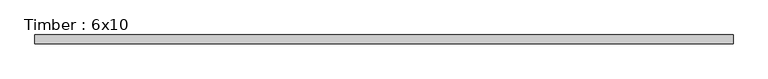
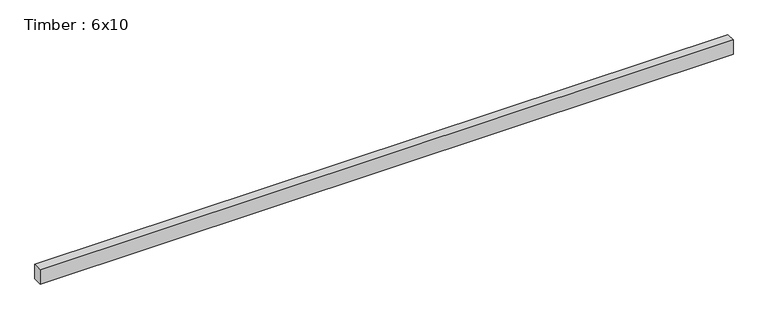
"""IFC4 building model written with IfcOpenShell, lengths in millimetres: beam geometry, Timber : 6x10."""

from ifc_helpers import new_model, si_unit, frame, origin, place, context, project, spatial, polyline, outline, extrude, source, transform, mapped, element, save


def timber_6x10_e342fa3e(model_context):
    return source(origin(), model_context, "Body", "SweptSolid", [
        extrude(outline(polyline([(5454.65, 69.85), (5454.65, -69.85), (-5454.65, -69.85), (-5454.65, 69.85), (5454.65, 69.85)])), frame((0.0, 0.0, -120.65), z_axis=(0.0, 0.0, 1.0), x_axis=(1.0, 0.0, 0.0)), (0.0, 0.0, 1.0), 241.3),
    ])


if __name__ == "__main__":
    model = new_model("IFC4")
    model_context = context("Model", 3, world=origin())
    ifc_project = project(units=[si_unit("LENGTHUNIT", "METRE", prefix="MILLI")], contexts=[model_context])
    site = spatial("IfcSite", under=ifc_project)
    building = spatial("IfcBuilding", under=site)
    placement = place(None, origin())
    timber_6x10_shape = timber_6x10_e342fa3e(model_context)
    element("IfcBeam", 1, ObjectType="Timber : 6x10", at=placement, inside=building, context=model_context, shape_type="MappedRepresentation", body=[
        mapped(timber_6x10_shape, transform((0.0, 0.0, 0.0), x_axis=(1.0, 0.0, 0.0), y_axis=(0.0, 1.0, 0.0), z_axis=(0.0, 0.0, 1.0))),
    ])
    save(model, "model.ifc")

# Revit data of these elements
# Type "Timber : 6x10"
#   Assembly Code = "B10"
#   A = 0.362847 SF
#   Length [instance default] = 5' - 0"
#   b = 0' - 5 1/2"
#   d = 0' - 9 1/2"
#   Structural Material [instance default] = Softwood, Lumber
# Element 1 (IfcBeam, "Timber : 6x10")
#   Materials on its faces: "Softwood, Lumber"
# Materials
#   "Softwood, Lumber": class "Wood", colour RGB 144 113 62, transparency 0, Description = "Pinus Echinata", Cost = 0
